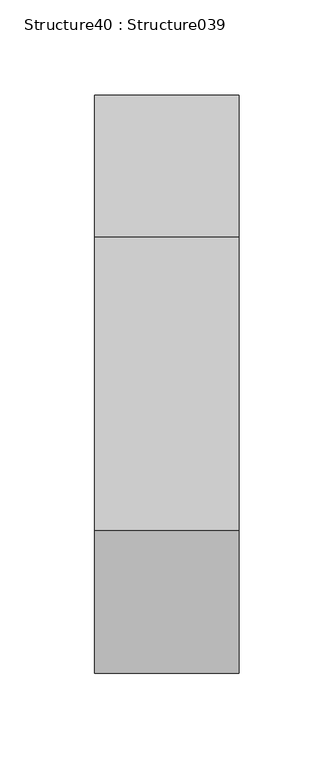
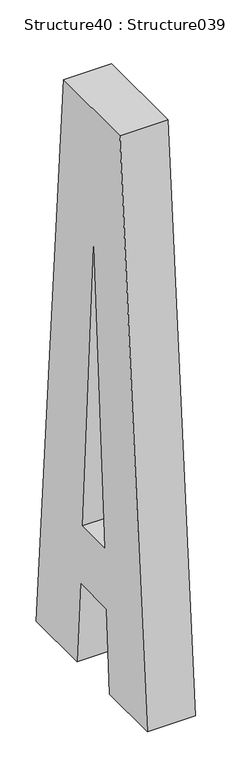
"""IFC4 building model written with IfcOpenShell, lengths in millimetres: proxy geometry, Structure40 : Structure039."""

from ifc_helpers import new_model, si_unit, frame, origin, place, context, project, spatial, polyline, outline, extrude, source, transform, mapped, element, save


def structure40_structure039_3784c563(model_context):
    return source(origin(), model_context, "Body", "SweptSolid", [
        extrude(outline(polyline([(249469.8898573, 3528.5825142), (249544.6793877, 4480.4419946), (249699.6997942, 4480.4419946), (249774.4798779, 3528.5825142), (249662.9896056, 3528.5825142), (249653.4609532, 3665.9109904), (249581.3857976, 3665.9109904), (249573.2407835, 3528.5825142), (249469.8898573, 3528.5825142)]), holes=[polyline([(249586.8328111, 3765.1859458), (249648.0208672, 3765.1859458), (249616.7539135, 4250.6490619), (249586.8328111, 3765.1859458)])]), frame((-38594.2176606, 0.0, 0.0), z_axis=(1.0, 0.0, 0.0), x_axis=(0.0, 1.0, 0.0)), (0.0, 0.0, 1.0), 76.2),
    ])


if __name__ == "__main__":
    model = new_model("IFC4")
    model_context = context("Model", 3, world=origin())
    ifc_project = project(units=[si_unit("LENGTHUNIT", "METRE", prefix="MILLI")], contexts=[model_context])
    site = spatial("IfcSite", under=ifc_project)
    building = spatial("IfcBuilding", under=site)
    placement = place(None, origin())
    structure40_structure039_shape = structure40_structure039_3784c563(model_context)
    element("IfcBuildingElementProxy", 1, Name="Structure40 : Structure039", ObjectType="Structure40 : Structure039", at=placement, inside=building, context=model_context, shape_type="MappedRepresentation", body=[
        mapped(structure40_structure039_shape, transform((0.0, 0.0, 0.0), x_axis=(1.0, 0.0, 0.0), y_axis=(0.0, 1.0, 0.0), z_axis=(0.0, 0.0, 1.0))),
    ])
    save(model, "model.ifc")

# Revit data of these elements
# Type "Structure40 : Structure039"
#   NameOverride = "Structure039"
# Element 1 (IfcBuildingElementProxy, "Structure40 : Structure039")
#   Materials on its faces: "BRUSHED ALUM. LETTERING"
# Materials
#   "BRUSHED ALUM. LETTERING": class "Unassigned", colour RGB 169 181 186, transparency 0, Cost = 0
